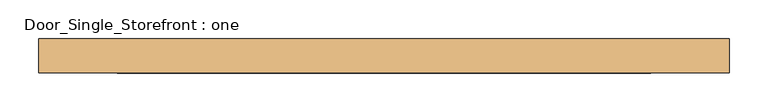
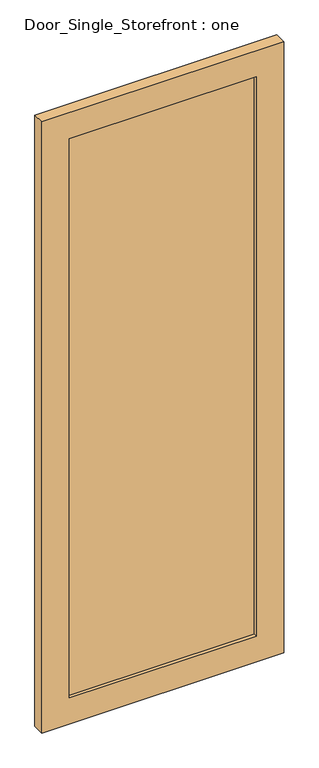
"""IFC4 building model written with IfcOpenShell, lengths in millimetres: door geometry, Door_Single_Storefront : one."""

import ifcopenshell
import ifcopenshell.guid

model = None  # the IFC model being written
_history = None  # IfcOwnerHistory: only IFC2X3 demands one
_inside = {}  # id of a spatial element -> (the spatial element, [elements in it])
_under = {}  # id of a project, library or spatial element -> (it, [spatial elements below it])
_declared = {}  # id of a project -> (the project, [libraries it declares])
_typed = {}  # id of a type object -> (the type object, [elements of that type])
_made_of = {}  # id of a material, layer set ... -> (it, [elements and type objects made of it])


def new_model(schema):
    """Start an empty IFC model of exactly this schema.

    Asked for "IFC4X3", IfcOpenShell would pick the latest addendum, in which some entities
    have other attributes; the version numbers below select the first issue.
    IFC2X3 requires an IfcOwnerHistory on every rooted entity: one is made here for all.
    """
    global model, _history
    if schema == "IFC4X3":
        model = ifcopenshell.file(schema_version=(4, 3, 0, 0))
    else:
        model = ifcopenshell.file(schema=schema)
    _inside.clear()
    _under.clear()
    _declared.clear()
    _typed.clear()
    _made_of.clear()
    _history = None
    if model.schema == "IFC2X3":
        org = make("IfcOrganization", Name="unknown")
        user = make(
            "IfcPersonAndOrganization",
            ThePerson=make("IfcPerson", FamilyName="unknown"),
            TheOrganization=org,
        )
        app = make(
            "IfcApplication",
            ApplicationDeveloper=org,
            Version="unknown",
            ApplicationFullName="unknown",
            ApplicationIdentifier="unknown",
        )
        _history = make(
            "IfcOwnerHistory",
            OwningUser=user,
            OwningApplication=app,
            ChangeAction="ADDED",
            CreationDate=0,
        )
    return model


def make(cls, **values):
    """One entity of the class cls with the attributes given. An attribute that is None is left unset."""
    return model.create_entity(
        cls, **{name: value for name, value in values.items() if value is not None}
    )


def rooted(cls, **values):
    """An entity with a GlobalId (a new one), such as an element, a storey or a relation."""
    return make(cls, GlobalId=ifcopenshell.guid.new(), OwnerHistory=_history, **values)


def si_unit(unit_type, name, prefix=None):
    """IfcSIUnit, for example si_unit("LENGTHUNIT", "METRE", prefix="MILLI")."""
    return make("IfcSIUnit", UnitType=unit_type, Prefix=prefix, Name=name)


def assignment(units):
    """IfcUnitAssignment: the units of a project."""
    return None if units is None else make("IfcUnitAssignment", Units=units)


def point(xyz):
    """IfcCartesianPoint."""
    return None if xyz is None else make("IfcCartesianPoint", Coordinates=xyz)


def direction(xyz):
    """IfcDirection."""
    return None if xyz is None else make("IfcDirection", DirectionRatios=xyz)


def frame(location, z_axis=None, x_axis=None):
    """IfcAxis2Placement3D, a coordinate frame: its origin and axes. An axis left out is left unset."""
    return make(
        "IfcAxis2Placement3D",
        Location=point(location),
        Axis=direction(z_axis),
        RefDirection=direction(x_axis),
    )


def origin():
    """The frame at (0, 0, 0) with its axes left unset."""
    return frame((0.0, 0.0, 0.0))


def place(relative_to, where):
    """IfcLocalPlacement: puts the frame where relative to a parent placement (None: the world)."""
    return make(
        "IfcLocalPlacement", PlacementRelTo=relative_to, RelativePlacement=where
    )


def context(
    kind, dimensions, precision=None, world=None, true_north=None, identifier=None
):
    """IfcGeometricRepresentationContext, for example the 3D "Model" context."""
    return make(
        "IfcGeometricRepresentationContext",
        ContextIdentifier=identifier,
        ContextType=kind,
        CoordinateSpaceDimension=dimensions,
        Precision=precision,
        WorldCoordinateSystem=world,
        TrueNorth=true_north,
    )


def project(units=None, contexts=None):
    """IfcProject with its units and contexts."""
    return rooted(
        "IfcProject",
        Name="project",
        RepresentationContexts=contexts,
        UnitsInContext=assignment(units),
    )


def spatial(cls, under=None, at=None, **own):
    """A site, building, storey or space (cls), placed at a placement, below another one or the project."""
    s = rooted(cls, ObjectPlacement=at, **own)
    if under is not None:
        _under.setdefault(under.id(), (under, []))[1].append(s)
    return s


def polyline(points):
    """IfcPolyline through the points."""
    return make("IfcPolyline", Points=[point(p) for p in points])


def outline(outer, holes=None, kind="AREA"):
    """IfcArbitraryClosedProfileDef: a profile drawn as a closed curve; with holes, ...WithVoids."""
    if holes is None:
        return make("IfcArbitraryClosedProfileDef", ProfileType=kind, OuterCurve=outer)
    return make(
        "IfcArbitraryProfileDefWithVoids",
        ProfileType=kind,
        OuterCurve=outer,
        InnerCurves=holes,
    )


def extrude(swept, where, along, depth):
    """IfcExtrudedAreaSolid: the profile swept, set in the frame where, extruded along a direction by depth."""
    return make(
        "IfcExtrudedAreaSolid",
        SweptArea=swept,
        Position=where,
        ExtrudedDirection=direction(along),
        Depth=depth,
    )


def shape(context_of_items, identifier, shape_type, items):
    """IfcShapeRepresentation: the items that make up one representation, for example the "Body"."""
    return make(
        "IfcShapeRepresentation",
        ContextOfItems=context_of_items,
        RepresentationIdentifier=identifier,
        RepresentationType=shape_type,
        Items=items,
    )


def source(mapping_origin, context_of_items, identifier, shape_type, items):
    """IfcRepresentationMap: a shape defined once, which mapped items show again and again."""
    return make(
        "IfcRepresentationMap",
        MappingOrigin=mapping_origin,
        MappedRepresentation=shape(context_of_items, identifier, shape_type, items),
    )


def transform(
    local_origin,
    x_axis=None,
    y_axis=None,
    z_axis=None,
    scale=None,
    scale2=None,
    scale3=None,
    uniform=True,
):
    """IfcCartesianTransformationOperator3D, or its non-uniform kind. x_axis, y_axis, z_axis: its Axis1, 2, 3."""
    if uniform:
        return make(
            "IfcCartesianTransformationOperator3D",
            Axis1=direction(x_axis),
            Axis2=direction(y_axis),
            LocalOrigin=point(local_origin),
            Scale=scale,
            Axis3=direction(z_axis),
        )
    return make(
        "IfcCartesianTransformationOperator3DnonUniform",
        Axis1=direction(x_axis),
        Axis2=direction(y_axis),
        LocalOrigin=point(local_origin),
        Scale=scale,
        Axis3=direction(z_axis),
        Scale2=scale2,
        Scale3=scale3,
    )


def mapped(mapping_source, mapping_target):
    """IfcMappedItem: shows the shape of a source again, moved by a transform."""
    return make(
        "IfcMappedItem", MappingSource=mapping_source, MappingTarget=mapping_target
    )


def made_of(thing, what):
    """Note that an element or type object is made of a material, layer set ...; save() writes the relation."""
    if what is not None:
        _made_of.setdefault(what.id(), (what, []))[1].append(thing)
    return thing


def element(
    cls,
    number,
    at=None,
    inside=None,
    cuts=None,
    type_object=None,
    material=None,
    context=None,
    identifier="Body",
    shape_type=None,
    held_by="IfcProductDefinitionShape",
    body=None,
    shapes=None,
    **own,
):
    """One element of the class cls, such as IfcWall. Its Tag is "e" and its number.

    at: its placement. inside: the storey or other place that contains it. cuts: it is an
    opening in that element (IfcRelVoidsElement). A single representation is given by context,
    identifier, shape_type and body (its items); several are given by shapes. held_by: the class
    of the entity that holds the representations. save() writes the other relations.
    """
    e = rooted(cls, Tag="e%d" % number, ObjectPlacement=at, **own)
    if body is not None:
        shapes = [shape(context, identifier, shape_type, body)]
    if shapes is not None:
        e.Representation = make(held_by, Representations=shapes)
    if inside is not None:
        _inside.setdefault(inside.id(), (inside, []))[1].append(e)
    if cuts is not None:
        rooted(
            "IfcRelVoidsElement", RelatingBuildingElement=cuts, RelatedOpeningElement=e
        )
    if type_object is not None:
        _typed.setdefault(type_object.id(), (type_object, []))[1].append(e)
    return made_of(e, material)


def aggregate(whole, parts):
    """IfcRelAggregates: a whole, such as a stair, and the parts it consists of."""
    return rooted("IfcRelAggregates", RelatingObject=whole, RelatedObjects=parts)


def save(model, path):
    """Write the relations noted so far, then the file.

    IfcRelAggregates (storeys below a building ...), IfcRelContainedInSpatialStructure (elements
    in a storey), IfcRelDefinesByType, IfcRelAssociatesMaterial and IfcRelDeclares: one each for
    every whole, place, type object, material and project.
    """
    for whole, parts in _under.values():
        aggregate(whole, parts)
    for where, things in _inside.values():
        rooted(
            "IfcRelContainedInSpatialStructure",
            RelatedElements=things,
            RelatingStructure=where,
        )
    for kind, things in _typed.values():
        rooted("IfcRelDefinesByType", RelatedObjects=things, RelatingType=kind)
    for what, things in _made_of.values():
        rooted("IfcRelAssociatesMaterial", RelatedObjects=things, RelatingMaterial=what)
    for by, libraries in _declared.values():
        rooted("IfcRelDeclares", RelatingContext=by, RelatedDefinitions=libraries)
    model.write(path)


def door_single_storefront_one_d1ec06f1(model_context):
    return source(origin(), model_context, "Body", "SweptSolid", [
        extrude(outline(polyline([(2387.6, -446.88125), (0.0, -446.88125), (0.0, 446.88125), (2387.6, 446.88125), (2387.6, -446.88125)]), holes=[polyline([(101.6, 345.28125), (101.6, -345.28125), (2286.0, -345.28125), (2286.0, 345.28125), (101.6, 345.28125)])]), frame((0.0, -50.8, 0.0), z_axis=(0.0, 1.0, 0.0), x_axis=(0.0, 0.0, 1.0)), (0.0, 0.0, 1.0), 44.45),
        extrude(outline(polyline([(345.28125, -19.05), (345.28125, -38.1), (-345.28125, -38.1), (-345.28125, -19.05), (345.28125, -19.05)])), frame((0.0, 0.0, 101.6), z_axis=(0.0, 0.0, 1.0), x_axis=(1.0, 0.0, 0.0)), (0.0, 0.0, 1.0), 2184.4),
    ])


if __name__ == "__main__":
    model = new_model("IFC4")
    model_context = context("Model", 3, world=origin())
    ifc_project = project(units=[si_unit("LENGTHUNIT", "METRE", prefix="MILLI")], contexts=[model_context])
    site = spatial("IfcSite", under=ifc_project)
    building = spatial("IfcBuilding", under=site)
    placement = place(None, origin())
    door_single_storefront_one_shape = door_single_storefront_one_d1ec06f1(model_context)
    element("IfcDoor", 1, ObjectType="Door_Single_Storefront : one", at=placement, inside=building, context=model_context, shape_type="MappedRepresentation", body=[
        mapped(door_single_storefront_one_shape, transform((0.0, 0.0, 0.0), x_axis=(1.0, 0.0, 0.0), y_axis=(0.0, 1.0, 0.0), z_axis=(0.0, 0.0, 1.0))),
    ])
    save(model, "model.ifc")

# Revit data of these elements
# Type "Door_Single_Storefront : one"
#   Type Mark = "27"
#   Analytic Construction = "<None>"
#   Stile_Width = 0' - 4"
#   Door_Thickness = 0' - 1 3/4"
#   Door_Offset = 0' - 2"
#   Glass_Material = Glass
#   Frame_Material = Aluminum
#   Function = (empty or 0)
# Element 1 (IfcDoor, "Door_Single_Storefront : one")
#   Materials on its faces: "Aluminum", "Glass"
# Materials
#   "Glass": class "Glass", colour RGB 0 128 192, transparency 0.75, Description = "Soda Lime Glass", Cost = 0
#   "Aluminum": class "Metal", colour RGB 247 247 247, transparency 0, Description = "Aluminum 6061", Cost = 0
